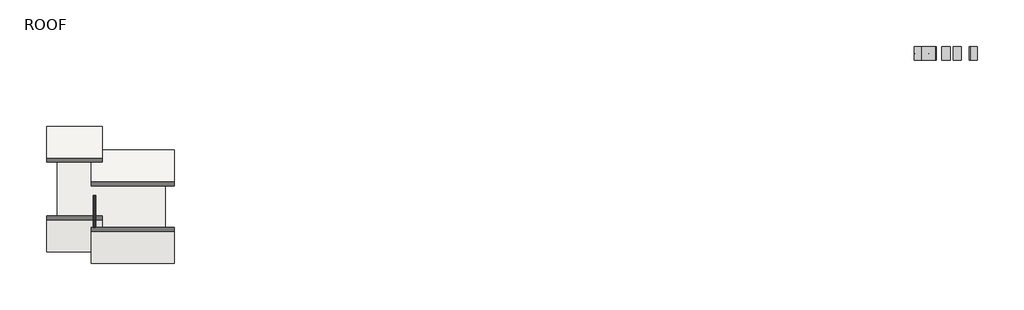
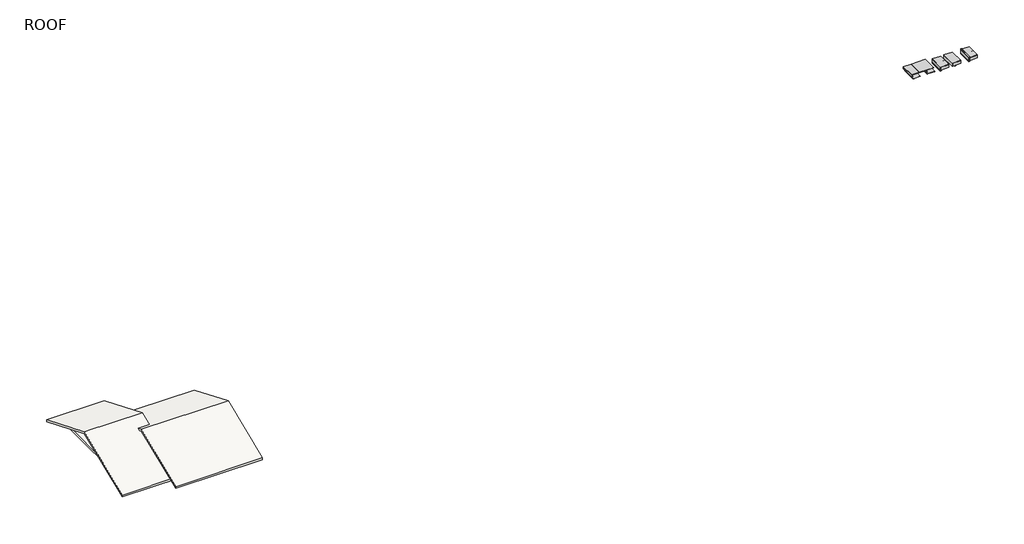
# One storey: 38 proxies, 2 roofs, 1 covering, 1 wall.
"""IFC4 building model written with IfcOpenShell, lengths in millimetres."""

import ifcopenshell
import ifcopenshell.guid

model = None  # the IFC model being written
_history = None  # IfcOwnerHistory: only IFC2X3 demands one
_inside = {}  # id of a spatial element -> (the spatial element, [elements in it])
_under = {}  # id of a project, library or spatial element -> (it, [spatial elements below it])
_declared = {}  # id of a project -> (the project, [libraries it declares])
_typed = {}  # id of a type object -> (the type object, [elements of that type])
_made_of = {}  # id of a material, layer set ... -> (it, [elements and type objects made of it])


def new_model(schema):
    """Start an empty IFC model of exactly this schema.

    Asked for "IFC4X3", IfcOpenShell would pick the latest addendum, in which some entities
    have other attributes; the version numbers below select the first issue.
    IFC2X3 requires an IfcOwnerHistory on every rooted entity: one is made here for all.
    """
    global model, _history
    if schema == "IFC4X3":
        model = ifcopenshell.file(schema_version=(4, 3, 0, 0))
    else:
        model = ifcopenshell.file(schema=schema)
    _inside.clear()
    _under.clear()
    _declared.clear()
    _typed.clear()
    _made_of.clear()
    _history = None
    if model.schema == "IFC2X3":
        org = make("IfcOrganization", Name="unknown")
        user = make(
            "IfcPersonAndOrganization",
            ThePerson=make("IfcPerson", FamilyName="unknown"),
            TheOrganization=org,
        )
        app = make(
            "IfcApplication",
            ApplicationDeveloper=org,
            Version="unknown",
            ApplicationFullName="unknown",
            ApplicationIdentifier="unknown",
        )
        _history = make(
            "IfcOwnerHistory",
            OwningUser=user,
            OwningApplication=app,
            ChangeAction="ADDED",
            CreationDate=0,
        )
    return model


def make(cls, **values):
    """One entity of the class cls with the attributes given. An attribute that is None is left unset."""
    return model.create_entity(
        cls, **{name: value for name, value in values.items() if value is not None}
    )


def rooted(cls, **values):
    """An entity with a GlobalId (a new one), such as an element, a storey or a relation."""
    return make(cls, GlobalId=ifcopenshell.guid.new(), OwnerHistory=_history, **values)


def si_unit(unit_type, name, prefix=None):
    """IfcSIUnit, for example si_unit("LENGTHUNIT", "METRE", prefix="MILLI")."""
    return make("IfcSIUnit", UnitType=unit_type, Prefix=prefix, Name=name)


def assignment(units):
    """IfcUnitAssignment: the units of a project."""
    return None if units is None else make("IfcUnitAssignment", Units=units)


def point(xyz):
    """IfcCartesianPoint."""
    return None if xyz is None else make("IfcCartesianPoint", Coordinates=xyz)


def direction(xyz):
    """IfcDirection."""
    return None if xyz is None else make("IfcDirection", DirectionRatios=xyz)


def frame(location, z_axis=None, x_axis=None):
    """IfcAxis2Placement3D, a coordinate frame: its origin and axes. An axis left out is left unset."""
    return make(
        "IfcAxis2Placement3D",
        Location=point(location),
        Axis=direction(z_axis),
        RefDirection=direction(x_axis),
    )


def origin():
    """The frame at (0, 0, 0) with its axes left unset."""
    return frame((0.0, 0.0, 0.0))


def place(relative_to, where):
    """IfcLocalPlacement: puts the frame where relative to a parent placement (None: the world)."""
    return make(
        "IfcLocalPlacement", PlacementRelTo=relative_to, RelativePlacement=where
    )


def context(
    kind, dimensions, precision=None, world=None, true_north=None, identifier=None
):
    """IfcGeometricRepresentationContext, for example the 3D "Model" context."""
    return make(
        "IfcGeometricRepresentationContext",
        ContextIdentifier=identifier,
        ContextType=kind,
        CoordinateSpaceDimension=dimensions,
        Precision=precision,
        WorldCoordinateSystem=world,
        TrueNorth=true_north,
    )


def project(units=None, contexts=None):
    """IfcProject with its units and contexts."""
    return rooted(
        "IfcProject",
        Name="project",
        RepresentationContexts=contexts,
        UnitsInContext=assignment(units),
    )


def spatial(cls, under=None, at=None, **own):
    """A site, building, storey or space (cls), placed at a placement, below another one or the project."""
    s = rooted(cls, ObjectPlacement=at, **own)
    if under is not None:
        _under.setdefault(under.id(), (under, []))[1].append(s)
    return s


def polyline(points):
    """IfcPolyline through the points."""
    return make("IfcPolyline", Points=[point(p) for p in points])


def outline(outer, holes=None, kind="AREA"):
    """IfcArbitraryClosedProfileDef: a profile drawn as a closed curve; with holes, ...WithVoids."""
    if holes is None:
        return make("IfcArbitraryClosedProfileDef", ProfileType=kind, OuterCurve=outer)
    return make(
        "IfcArbitraryProfileDefWithVoids",
        ProfileType=kind,
        OuterCurve=outer,
        InnerCurves=holes,
    )


def extrude(swept, where, along, depth):
    """IfcExtrudedAreaSolid: the profile swept, set in the frame where, extruded along a direction by depth."""
    return make(
        "IfcExtrudedAreaSolid",
        SweptArea=swept,
        Position=where,
        ExtrudedDirection=direction(along),
        Depth=depth,
    )


def shape(context_of_items, identifier, shape_type, items):
    """IfcShapeRepresentation: the items that make up one representation, for example the "Body"."""
    return make(
        "IfcShapeRepresentation",
        ContextOfItems=context_of_items,
        RepresentationIdentifier=identifier,
        RepresentationType=shape_type,
        Items=items,
    )


def source(mapping_origin, context_of_items, identifier, shape_type, items):
    """IfcRepresentationMap: a shape defined once, which mapped items show again and again."""
    return make(
        "IfcRepresentationMap",
        MappingOrigin=mapping_origin,
        MappedRepresentation=shape(context_of_items, identifier, shape_type, items),
    )


def transform(
    local_origin,
    x_axis=None,
    y_axis=None,
    z_axis=None,
    scale=None,
    scale2=None,
    scale3=None,
    uniform=True,
):
    """IfcCartesianTransformationOperator3D, or its non-uniform kind. x_axis, y_axis, z_axis: its Axis1, 2, 3."""
    if uniform:
        return make(
            "IfcCartesianTransformationOperator3D",
            Axis1=direction(x_axis),
            Axis2=direction(y_axis),
            LocalOrigin=point(local_origin),
            Scale=scale,
            Axis3=direction(z_axis),
        )
    return make(
        "IfcCartesianTransformationOperator3DnonUniform",
        Axis1=direction(x_axis),
        Axis2=direction(y_axis),
        LocalOrigin=point(local_origin),
        Scale=scale,
        Axis3=direction(z_axis),
        Scale2=scale2,
        Scale3=scale3,
    )


def mapped(mapping_source, mapping_target):
    """IfcMappedItem: shows the shape of a source again, moved by a transform."""
    return make(
        "IfcMappedItem", MappingSource=mapping_source, MappingTarget=mapping_target
    )


def made_of(thing, what):
    """Note that an element or type object is made of a material, layer set ...; save() writes the relation."""
    if what is not None:
        _made_of.setdefault(what.id(), (what, []))[1].append(thing)
    return thing


def element(
    cls,
    number,
    at=None,
    inside=None,
    cuts=None,
    type_object=None,
    material=None,
    context=None,
    identifier="Body",
    shape_type=None,
    held_by="IfcProductDefinitionShape",
    body=None,
    shapes=None,
    **own,
):
    """One element of the class cls, such as IfcWall. Its Tag is "e" and its number.

    at: its placement. inside: the storey or other place that contains it. cuts: it is an
    opening in that element (IfcRelVoidsElement). A single representation is given by context,
    identifier, shape_type and body (its items); several are given by shapes. held_by: the class
    of the entity that holds the representations. save() writes the other relations.
    """
    e = rooted(cls, Tag="e%d" % number, ObjectPlacement=at, **own)
    if body is not None:
        shapes = [shape(context, identifier, shape_type, body)]
    if shapes is not None:
        e.Representation = make(held_by, Representations=shapes)
    if inside is not None:
        _inside.setdefault(inside.id(), (inside, []))[1].append(e)
    if cuts is not None:
        rooted(
            "IfcRelVoidsElement", RelatingBuildingElement=cuts, RelatedOpeningElement=e
        )
    if type_object is not None:
        _typed.setdefault(type_object.id(), (type_object, []))[1].append(e)
    return made_of(e, material)


def aggregate(whole, parts):
    """IfcRelAggregates: a whole, such as a stair, and the parts it consists of."""
    return rooted("IfcRelAggregates", RelatingObject=whole, RelatedObjects=parts)


def save(model, path):
    """Write the relations noted so far, then the file.

    IfcRelAggregates (storeys below a building ...), IfcRelContainedInSpatialStructure (elements
    in a storey), IfcRelDefinesByType, IfcRelAssociatesMaterial and IfcRelDeclares: one each for
    every whole, place, type object, material and project.
    """
    for whole, parts in _under.values():
        aggregate(whole, parts)
    for where, things in _inside.values():
        rooted(
            "IfcRelContainedInSpatialStructure",
            RelatedElements=things,
            RelatingStructure=where,
        )
    for kind, things in _typed.values():
        rooted("IfcRelDefinesByType", RelatedObjects=things, RelatingType=kind)
    for what, things in _made_of.values():
        rooted("IfcRelAssociatesMaterial", RelatedObjects=things, RelatingMaterial=what)
    for by, libraries in _declared.values():
        rooted("IfcRelDeclares", RelatingContext=by, RelatedDefinitions=libraries)
    model.write(path)


def generic_models_10_generic_models_1_ea081297(model_context):
    return source(origin(), model_context, "Body", "SweptSolid", [
        extrude(outline(polyline([(49758.6, 0.0), (49720.5, 0.0), (49720.5, 1219.2), (49758.6, 1219.2), (49758.6, 0.0)])), frame((0.0, 0.0, 5507.83125), z_axis=(0.0, 0.0, 1.0), x_axis=(1.0, 0.0, 0.0)), (0.0, 0.0, 1.0), 139.7),
    ])


def generic_models_109_generic_models_1_8619d77b(model_context):
    return source(origin(), model_context, "Body", "SweptSolid", [
        extrude(outline(polyline([(51003.2, 0.0), (50914.3, 0.0), (50914.3, 1219.2), (51003.2, 1219.2), (51003.2, 0.0)])), frame((0.0, 0.0, 5184.378125), z_axis=(0.0, 0.0, 1.0), x_axis=(1.0, 0.0, 0.0)), (0.0, 0.0, 1.0), 38.1),
    ])


def generic_models_110_generic_models_1_6bdce9b6(model_context):
    return source(origin(), model_context, "Body", "SweptSolid", [
        extrude(outline(polyline([(51642.1451407, 1219.2), (51642.1451407, 0.0), (50914.3, 0.0), (50914.3, 1219.2), (51642.1451407, 1219.2)])), frame((0.0, 0.0, 5508.228125), z_axis=(0.0, 0.0, 1.0), x_axis=(1.0, 0.0, 0.0)), (0.0, 0.0, 1.0), 19.05),
    ])


def generic_models_112_generic_models_65_d168d7b0(model_context):
    return source(origin(), model_context, "Body", "SweptSolid", [
        extrude(outline(polyline([(50952.4, 592.1375), (50952.4, 630.2375), (51642.1451407, 630.2375), (51642.1451407, 592.1375), (50952.4, 592.1375)])), frame((0.0, 0.0, 5222.478125), z_axis=(0.0, 0.0, 1.0), x_axis=(1.0, 0.0, 0.0)), (0.0, 0.0, 1.0), 285.75),
    ])


def generic_models_113_generic_models_1_101608ab(model_context):
    return source(origin(), model_context, "Body", "SweptSolid", [
        extrude(outline(polyline([(52171.6, 0.0), (52133.5, 0.0), (52133.5, 1219.2), (52171.6, 1219.2), (52171.6, 0.0)])), frame((0.0, 0.0, 5222.478125), z_axis=(0.0, 0.0, 1.0), x_axis=(1.0, 0.0, 0.0)), (0.0, 0.0, 1.0), 285.75),
    ])


def generic_models_114_generic_models_1_a6fb1c2c(model_context):
    return source(origin(), model_context, "Body", "SweptSolid", [
        extrude(outline(polyline([(51642.1451407, 1219.2), (51642.1451407, 0.0), (50965.9242022, 0.0), (50965.9242022, 1219.2), (51642.1451407, 1219.2)])), frame((0.0, 0.0, 5237.6235034), z_axis=(0.0, 0.0, 1.0), x_axis=(1.0, 0.0, 0.0)), (0.0, 0.0, 1.0), 254.0),
    ])


def generic_models_12_generic_models_46_b8a9a4e8(model_context):
    return source(origin(), model_context, "Body", "SweptSolid", [
        extrude(outline(polyline([(49757.8505137, 0.0), (49721.1284797, 0.0), (49721.1284797, 1219.2), (49757.8505137, 1219.2), (49757.8505137, 0.0)])), frame((0.0, 0.0, 5505.7509163), z_axis=(0.0, 0.0, 1.0), x_axis=(1.0, 0.0, 0.0)), (0.0, 0.0, 1.0), 1.5875),
    ])


def generic_models_13_generic_models_65_9e643fb9(model_context):
    return source(origin(), model_context, "Body", "SweptSolid", [
        extrude(outline(polyline([(49128.3625, 592.1375), (49128.3625, 630.2375), (50347.5625, 630.2375), (50347.5625, 592.1375), (49128.3625, 592.1375)])), frame((0.0, 0.0, 5507.83125), z_axis=(0.0, 0.0, 1.0), x_axis=(1.0, 0.0, 0.0)), (0.0, 0.0, 1.0), 139.7),
    ])


def generic_models_14_generic_models_1_e8c90d4c(model_context):
    return source(origin(), model_context, "Body", "SweptSolid", [
        extrude(outline(polyline([(2277.1204978, 49799.875), (2239.0204978, 49799.875), (2239.0204978, 49825.275), (2240.6079978, 49825.275), (2240.6079978, 49801.4625), (2277.1204978, 49801.4625), (2277.1204978, 49799.875)])), frame((0.0, 0.0, 0.0), z_axis=(0.0, 1.0, 0.0), x_axis=(0.0, 0.0, 1.0)), (0.0, 0.0, 1.0), 1219.2),
    ])


def generic_models_22_generic_models_1_e5767157(model_context):
    return source(origin(), model_context, "Body", "SweptSolid", [
        extrude(outline(polyline([(2409.6091, 49800.66875), (2409.6091, 49799.875), (2407.0592364, 49799.875), (2405.4618473, 49749.075), (2404.6631527, 49749.075), (2403.0657636, 49799.875), (2400.5159, 49799.875), (2400.5159, 49800.66875), (2409.6091, 49800.66875)])), frame((0.0, 565.15, 0.0), z_axis=(0.0, 1.0, 0.0), x_axis=(0.0, 0.0, 1.0)), (0.0, 0.0, 1.0), 12.7),
    ])


def generic_models_226_generic_models_1_7dc37832(model_context):
    return source(origin(), model_context, "Body", "SweptSolid", [
        extrude(outline(polyline([(5263.35625, 49733.4159), (5263.35625, 49742.5091), (5264.15, 49742.5091), (5264.15, 49739.9592364), (5314.95, 49738.3618473), (5314.95, 49737.5631527), (5264.15, 49735.9657636), (5264.15, 49733.4159), (5263.35625, 49733.4159)])), frame((0.0, 565.15, 0.0), z_axis=(0.0, 1.0, 0.0), x_axis=(0.0, 0.0, 1.0)), (0.0, 0.0, 1.0), 12.7),
    ])


def generic_models_202_generic_models_1_0ad20a8b(model_context):
    return source(origin(), model_context, "Body", "SweptSolid", [
        extrude(outline(polyline([(2253.330428, 49813.3451407), (2242.217928, 49813.3451407), (2242.217928, 49826.0451407), (2234.280428, 49828.9341545), (2234.280428, 50422.9451407), (2253.330428, 50422.9451407), (2253.330428, 49813.3451407)])), frame((0.0, 0.0, 0.0), z_axis=(0.0, 1.0, 0.0), x_axis=(0.0, 0.0, 1.0)), (0.0, 0.0, 1.0), 1219.2),
    ])


def generic_models_233_generic_models_1_ae5bae41(model_context):
    return source(origin(), model_context, "Body", "SweptSolid", [
        extrude(outline(polyline([(48564.8, 0.0), (48475.9, 0.0), (48475.9, 1219.2), (48564.8, 1219.2), (48564.8, 0.0)])), frame((0.0, 0.0, 5467.35), z_axis=(0.0, 0.0, 1.0), x_axis=(1.0, 0.0, 0.0)), (0.0, 0.0, 1.0), 38.1),
    ])


def generic_models_236_generic_models_1_f8917e71(model_context):
    return source(origin(), model_context, "Body", "SweptSolid", [
        extrude(outline(polyline([(48507.65, 0.0), (48469.55, 0.0), (48469.55, 1219.2), (48507.65, 1219.2), (48507.65, 0.0)])), frame((0.0, 0.0, 5507.83125), z_axis=(0.0, 0.0, 1.0), x_axis=(1.0, 0.0, 0.0)), (0.0, 0.0, 1.0), 139.7),
    ])


def generic_models_237_generic_models_65_1df05f16(model_context):
    return source(origin(), model_context, "Body", "SweptSolid", [
        extrude(outline(polyline([(48469.55, 592.1375), (48469.55, 630.2375), (49128.3625, 630.2375), (49128.3625, 592.1375), (48469.55, 592.1375)])), frame((0.0, 0.0, 5507.83125), z_axis=(0.0, 0.0, 1.0), x_axis=(1.0, 0.0, 0.0)), (0.0, 0.0, 1.0), 139.7),
    ])


def generic_models_239_generic_models_46_95e6735a(model_context):
    return source(origin(), model_context, "Body", "SweptSolid", [
        extrude(outline(polyline([(50347.5625, 0.0), (49691.4320511, 0.0), (49691.4320511, 1219.2), (50347.5625, 1219.2), (50347.5625, 0.0)])), frame((0.0, 0.0, 5505.7509163), z_axis=(0.0, 0.0, 1.0), x_axis=(1.0, 0.0, 0.0)), (0.0, 0.0, 1.0), 1.5875),
    ])


def generic_models_240_generic_models_1_611786cf(model_context):
    return source(origin(), model_context, "Body", "SweptSolid", [
        extrude(outline(polyline([(49128.3625, 1219.2), (49128.3625, 0.0), (48469.55, 0.0), (48469.55, 1219.2), (49128.3625, 1219.2)])), frame((0.0, 0.0, 5649.9125), z_axis=(0.0, 0.0, 1.0), x_axis=(1.0, 0.0, 0.0)), (0.0, 0.0, 1.0), 19.05),
    ])


def generic_models_29_generic_models_1_59087225(model_context):
    return source(origin(), model_context, "Body", "SweptSolid", [
        extrude(outline(polyline([(50347.5625, 1219.2), (50347.5625, 0.0), (49128.3625, 0.0), (49128.3625, 1219.2), (50347.5625, 1219.2)])), frame((0.0, 0.0, 5647.53125), z_axis=(0.0, 0.0, 1.0), x_axis=(1.0, 0.0, 0.0)), (0.0, 0.0, 1.0), 19.05),
    ])


def generic_models_37_generic_models_1_916dd7c6(model_context):
    return source(origin(), model_context, "Body", "SweptSolid", [
        extrude(outline(polyline([(2409.6091, 49675.25625), (2400.5159, 49675.25625), (2400.5159, 49676.05), (2403.0657636, 49676.05), (2404.6631527, 49726.85), (2405.4618473, 49726.85), (2407.0592364, 49676.05), (2409.6091, 49676.05), (2409.6091, 49675.25625)])), frame((0.0, 565.15, 0.0), z_axis=(0.0, 1.0, 0.0), x_axis=(0.0, 0.0, 1.0)), (0.0, 0.0, 1.0), 12.7),
    ])


def generic_models_103_generic_models_1_250a6a11(model_context):
    return source(origin(), model_context, "Body", "SweptSolid", [
        extrude(outline(polyline([(49784.0, 0.0), (49695.1, 0.0), (49695.1, 1219.2), (49784.0, 1219.2), (49784.0, 0.0)])), frame((0.0, 0.0, 5264.15), z_axis=(0.0, 0.0, 1.0), x_axis=(1.0, 0.0, 0.0)), (0.0, 0.0, 1.0), 38.1),
    ])


def generic_models_71_generic_models_1_508a995f(model_context):
    return source(origin(), model_context, "Body", "SweptSolid", [
        extrude(outline(polyline([(50952.4, 0.0), (50914.3, 0.0), (50914.3, 1219.2), (50952.4, 1219.2), (50952.4, 0.0)])), frame((0.0, 0.0, 5222.478125), z_axis=(0.0, 0.0, 1.0), x_axis=(1.0, 0.0, 0.0)), (0.0, 0.0, 1.0), 285.75),
    ])


def generic_models_87_generic_models_1_55a64953(model_context):
    return source(origin(), model_context, "Body", "SweptSolid", [
        extrude(outline(polyline([(51968.4, 0.0), (51930.3, 0.0), (51930.3, 1219.2), (51968.4, 1219.2), (51968.4, 0.0)])), frame((0.0, 0.0, 5222.478125), z_axis=(0.0, 0.0, 1.0), x_axis=(1.0, 0.0, 0.0)), (0.0, 0.0, 1.0), 285.75),
    ])


model = new_model("IFC4")

# Units and contexts
model_context = context("Model", 3, world=origin())
ifc_project = project(units=[si_unit("LENGTHUNIT", "METRE", prefix="MILLI")], contexts=[model_context])

# Site, building, storey
site = spatial("IfcSite", under=ifc_project)
building = spatial("IfcBuilding", under=site)
storey = spatial("IfcBuildingStorey", under=building, Name="ROOF", Elevation=5130.8)

# Proxies
placement = place(None, origin())
generic_models_10_generic_models_1_shape = generic_models_10_generic_models_1_ea081297(model_context)
element("IfcBuildingElementProxy", 1, Name="Generic Models 10 : Generic Models 1", ObjectType="Generic Models 10 : Generic Models 1", at=placement, inside=storey, context=model_context, shape_type="MappedRepresentation", body=[
    mapped(generic_models_10_generic_models_1_shape, transform((0.0, 0.0, 0.0), x_axis=(1.0, 0.0, 0.0), y_axis=(0.0, 1.0, 0.0), z_axis=(0.0, 0.0, 1.0))),
])
generic_models_109_generic_models_1_shape = generic_models_109_generic_models_1_8619d77b(model_context)
element("IfcBuildingElementProxy", 2, Name="Generic Models 109 : Generic Models 1", ObjectType="Generic Models 109 : Generic Models 1", at=placement, inside=storey, context=model_context, shape_type="MappedRepresentation", body=[
    mapped(generic_models_109_generic_models_1_shape, transform((2438.4, 0.0, 0.0), x_axis=(1.0, 0.0, 0.0), y_axis=(0.0, 1.0, 0.0), z_axis=(0.0, 0.0, 1.0))),
])
generic_models_110_generic_models_1_shape = generic_models_110_generic_models_1_6bdce9b6(model_context)
element("IfcBuildingElementProxy", 3, Name="Generic Models 110 : Generic Models 1", ObjectType="Generic Models 110 : Generic Models 1", at=placement, inside=storey, context=model_context, shape_type="MappedRepresentation", body=[
    mapped(generic_models_110_generic_models_1_shape, transform((2438.4, 0.0, 0.0), x_axis=(1.0, 0.0, 0.0), y_axis=(0.0, 1.0, 0.0), z_axis=(0.0, 0.0, 1.0))),
])
element("IfcBuildingElementProxy", 4, Name="Generic Models 111 : Generic Models 1", ObjectType="Generic Models 111 : Generic Models 1", at=placement, inside=storey, context=model_context, shape_type="MappedRepresentation", body=[
    mapped(generic_models_109_generic_models_1_shape, transform((2438.4, 0.0, -38.1), x_axis=(1.0, 0.0, 0.0), y_axis=(0.0, 1.0, 0.0), z_axis=(0.0, 0.0, 1.0))),
])
generic_models_112_generic_models_65_shape = generic_models_112_generic_models_65_d168d7b0(model_context)
element("IfcBuildingElementProxy", 5, Name="Generic Models 112 : Generic Models 65", ObjectType="Generic Models 112 : Generic Models 65", at=placement, inside=storey, context=model_context, shape_type="MappedRepresentation", body=[
    mapped(generic_models_112_generic_models_65_shape, transform((2438.4, 0.0, 0.0), x_axis=(1.0, 0.0, 0.0), y_axis=(0.0, 1.0, 0.0), z_axis=(0.0, 0.0, 1.0))),
])
generic_models_113_generic_models_1_shape = generic_models_113_generic_models_1_101608ab(model_context)
element("IfcBuildingElementProxy", 6, Name="Generic Models 113 : Generic Models 1", ObjectType="Generic Models 113 : Generic Models 1", at=placement, inside=storey, context=model_context, shape_type="MappedRepresentation", body=[
    mapped(generic_models_113_generic_models_1_shape, transform((1219.2, 0.0, 0.0), x_axis=(1.0, 0.0, 0.0), y_axis=(0.0, 1.0, 0.0), z_axis=(0.0, 0.0, 1.0))),
])
generic_models_114_generic_models_1_shape = generic_models_114_generic_models_1_a6fb1c2c(model_context)
element("IfcBuildingElementProxy", 7, Name="Generic Models 114 : Generic Models 1", ObjectType="Generic Models 114 : Generic Models 1", at=placement, inside=storey, context=model_context, shape_type="MappedRepresentation", body=[
    mapped(generic_models_114_generic_models_1_shape, transform((2438.4, 0.0, 0.0), x_axis=(1.0, 0.0, 0.0), y_axis=(0.0, 1.0, 0.0), z_axis=(0.0, 0.0, 1.0))),
])
element("IfcBuildingElementProxy", 8, Name="Generic Models 115 : Generic Models 1", ObjectType="Generic Models 115 : Generic Models 1", at=placement, inside=storey, context=model_context, shape_type="MappedRepresentation", body=[
    mapped(generic_models_109_generic_models_1_shape, transform((2438.4, 0.0, 342.9), x_axis=(1.0, 0.0, 0.0), y_axis=(0.0, 1.0, 0.0), z_axis=(0.0, 0.0, 1.0))),
])
generic_models_12_generic_models_46_shape = generic_models_12_generic_models_46_b8a9a4e8(model_context)
element("IfcBuildingElementProxy", 9, Name="Generic Models 12 : Generic Models 46", ObjectType="Generic Models 12 : Generic Models 46", at=placement, inside=storey, context=model_context, shape_type="MappedRepresentation", body=[
    mapped(generic_models_12_generic_models_46_shape, transform((0.0, 0.0, 0.0), x_axis=(1.0, 0.0, 0.0), y_axis=(0.0, 1.0, 0.0), z_axis=(0.0, 0.0, 1.0))),
])
generic_models_13_generic_models_65_shape = generic_models_13_generic_models_65_9e643fb9(model_context)
element("IfcBuildingElementProxy", 10, Name="Generic Models 13 : Generic Models 65", ObjectType="Generic Models 13 : Generic Models 65", at=placement, inside=storey, context=model_context, shape_type="MappedRepresentation", body=[
    mapped(generic_models_13_generic_models_65_shape, transform((0.0, 0.0, 0.0), x_axis=(1.0, 0.0, 0.0), y_axis=(0.0, 1.0, 0.0), z_axis=(0.0, 0.0, 1.0))),
])
generic_models_14_generic_models_1_shape = generic_models_14_generic_models_1_e8c90d4c(model_context)
element("IfcBuildingElementProxy", 11, Name="Generic Models 14 : Generic Models 1", ObjectType="Generic Models 14 : Generic Models 1", at=placement, inside=storey, context=model_context, shape_type="MappedRepresentation", body=[
    mapped(generic_models_14_generic_models_1_shape, transform((0.0, 0.0, 3050.778125), x_axis=(1.0, 0.0, 0.0), y_axis=(0.0, 1.0, 0.0), z_axis=(0.0, 0.0, 1.0))),
])
generic_models_22_generic_models_1_shape = generic_models_22_generic_models_1_e5767157(model_context)
element("IfcBuildingElementProxy", 12, Name="Generic Models 22 : Generic Models 1", ObjectType="Generic Models 22 : Generic Models 1", at=placement, inside=storey, context=model_context, shape_type="MappedRepresentation", body=[
    mapped(generic_models_22_generic_models_1_shape, transform((0.0, 0.0, 3081.3375), x_axis=(1.0, 0.0, 0.0), y_axis=(0.0, 1.0, 0.0), z_axis=(0.0, 0.0, 1.0))),
])
element("IfcBuildingElementProxy", 13, Name="Generic Models 224 : Generic Models 1", ObjectType="Generic Models 224 : Generic Models 1", at=placement, inside=storey, context=model_context, shape_type="MappedRepresentation", body=[
    mapped(generic_models_14_generic_models_1_shape, transform((-1217.6125, 0.0, 3050.778125), x_axis=(1.0, 0.0, 0.0), y_axis=(0.0, 1.0, 0.0), z_axis=(0.0, 0.0, 1.0))),
])
element("IfcBuildingElementProxy", 14, Name="Generic Models 225 : Generic Models 1", ObjectType="Generic Models 225 : Generic Models 1", at=placement, inside=storey, context=model_context, shape_type="MappedRepresentation", body=[
    mapped(generic_models_22_generic_models_1_shape, transform((-1219.2, 0.0, 3081.3375), x_axis=(1.0, 0.0, 0.0), y_axis=(0.0, 1.0, 0.0), z_axis=(0.0, 0.0, 1.0))),
])
generic_models_226_generic_models_1_shape = generic_models_226_generic_models_1_7dc37832(model_context)
element("IfcBuildingElementProxy", 15, Name="Generic Models 226 : Generic Models 1", ObjectType="Generic Models 226 : Generic Models 1", at=placement, inside=storey, context=model_context, shape_type="MappedRepresentation", body=[
    mapped(generic_models_226_generic_models_1_shape, transform((-1219.2, 0.0, 203.2), x_axis=(1.0, 0.0, 0.0), y_axis=(0.0, 1.0, 0.0), z_axis=(0.0, 0.0, 1.0))),
])
generic_models_202_generic_models_1_shape = generic_models_202_generic_models_1_0ad20a8b(model_context)
element("IfcBuildingElementProxy", 16, Name="Generic Models 231 : Generic Models 1", ObjectType="Generic Models 231 : Generic Models 1", at=placement, inside=storey, context=model_context, shape_type="MappedRepresentation", body=[
    mapped(generic_models_202_generic_models_1_shape, transform((-1217.6125, 0.0, 3050.778125), x_axis=(1.0, 0.0, 0.0), y_axis=(0.0, 1.0, 0.0), z_axis=(0.0, 0.0, 1.0))),
])
generic_models_233_generic_models_1_shape = generic_models_233_generic_models_1_ae5bae41(model_context)
element("IfcBuildingElementProxy", 17, Name="Generic Models 233 : Generic Models 1", ObjectType="Generic Models 233 : Generic Models 1", at=placement, inside=storey, context=model_context, shape_type="MappedRepresentation", body=[
    mapped(generic_models_233_generic_models_1_shape, transform((0.0, 0.0, 0.0), x_axis=(1.0, 0.0, 0.0), y_axis=(0.0, 1.0, 0.0), z_axis=(0.0, 0.0, 1.0))),
])
generic_models_236_generic_models_1_shape = generic_models_236_generic_models_1_f8917e71(model_context)
element("IfcBuildingElementProxy", 18, Name="Generic Models 236 : Generic Models 1", ObjectType="Generic Models 236 : Generic Models 1", at=placement, inside=storey, context=model_context, shape_type="MappedRepresentation", body=[
    mapped(generic_models_236_generic_models_1_shape, transform((0.0, 0.0, 0.0), x_axis=(1.0, 0.0, 0.0), y_axis=(0.0, 1.0, 0.0), z_axis=(0.0, 0.0, 1.0))),
])
generic_models_237_generic_models_65_shape = generic_models_237_generic_models_65_1df05f16(model_context)
element("IfcBuildingElementProxy", 19, Name="Generic Models 237 : Generic Models 65", ObjectType="Generic Models 237 : Generic Models 65", at=placement, inside=storey, context=model_context, shape_type="MappedRepresentation", body=[
    mapped(generic_models_237_generic_models_65_shape, transform((0.0, 0.0, 0.0), x_axis=(1.0, 0.0, 0.0), y_axis=(0.0, 1.0, 0.0), z_axis=(0.0, 0.0, 1.0))),
])
generic_models_239_generic_models_46_shape = generic_models_239_generic_models_46_95e6735a(model_context)
element("IfcBuildingElementProxy", 20, Name="Generic Models 239 : Generic Models 46", ObjectType="Generic Models 239 : Generic Models 46", at=placement, inside=storey, context=model_context, shape_type="MappedRepresentation", body=[
    mapped(generic_models_239_generic_models_46_shape, transform((-1219.2, 0.0, 142.08125), x_axis=(1.0, 0.0, 0.0), y_axis=(0.0, 1.0, 0.0), z_axis=(0.0, 0.0, 1.0))),
])
generic_models_240_generic_models_1_shape = generic_models_240_generic_models_1_611786cf(model_context)
element("IfcBuildingElementProxy", 21, Name="Generic Models 240 : Generic Models 1", ObjectType="Generic Models 240 : Generic Models 1", at=placement, inside=storey, context=model_context, shape_type="MappedRepresentation", body=[
    mapped(generic_models_240_generic_models_1_shape, transform((0.0, 0.0, 0.0), x_axis=(1.0, 0.0, 0.0), y_axis=(0.0, 1.0, 0.0), z_axis=(0.0, 0.0, 1.0))),
])
element("IfcBuildingElementProxy", 22, Name="Generic Models 25 : Generic Models 46", ObjectType="Generic Models 25 : Generic Models 46", at=placement, inside=storey, context=model_context, shape_type="MappedRepresentation", body=[
    mapped(generic_models_12_generic_models_46_shape, transform((0.0, 0.0, 142.08125), x_axis=(1.0, 0.0, 0.0), y_axis=(0.0, 1.0, 0.0), z_axis=(0.0, 0.0, 1.0))),
])
generic_models_29_generic_models_1_shape = generic_models_29_generic_models_1_59087225(model_context)
element("IfcBuildingElementProxy", 23, Name="Generic Models 29 : Generic Models 1", ObjectType="Generic Models 29 : Generic Models 1", at=placement, inside=storey, context=model_context, shape_type="MappedRepresentation", body=[
    mapped(generic_models_29_generic_models_1_shape, transform((0.0, 0.0, 2.38125), x_axis=(1.0, 0.0, 0.0), y_axis=(0.0, 1.0, 0.0), z_axis=(0.0, 0.0, 1.0))),
])
element("IfcBuildingElementProxy", 24, Name="Generic Models 39 : Generic Models 1", ObjectType="Generic Models 39 : Generic Models 1", at=placement, inside=storey, context=model_context, shape_type="MappedRepresentation", body=[
    mapped(generic_models_226_generic_models_1_shape, transform((0.0, 0.0, 203.2), x_axis=(1.0, 0.0, 0.0), y_axis=(0.0, 1.0, 0.0), z_axis=(0.0, 0.0, 1.0))),
])
generic_models_37_generic_models_1_shape = generic_models_37_generic_models_1_916dd7c6(model_context)
element("IfcBuildingElementProxy", 25, Name="Generic Models 47 : Generic Models 1", ObjectType="Generic Models 47 : Generic Models 1", at=placement, inside=storey, context=model_context, shape_type="MappedRepresentation", body=[
    mapped(generic_models_37_generic_models_1_shape, transform((3.175, 0.0, 3081.3375), x_axis=(1.0, 0.0, 0.0), y_axis=(0.0, 1.0, 0.0), z_axis=(0.0, 0.0, 1.0))),
])
element("IfcBuildingElementProxy", 26, Name="Generic Models 49 : Generic Models 1", ObjectType="Generic Models 49 : Generic Models 1", at=placement, inside=storey, context=model_context, shape_type="MappedRepresentation", body=[
    mapped(generic_models_202_generic_models_1_shape, transform((0.0, 0.0, 3050.778125), x_axis=(1.0, 0.0, 0.0), y_axis=(0.0, 1.0, 0.0), z_axis=(0.0, 0.0, 1.0))),
])
element("IfcBuildingElementProxy", 27, Name="Generic Models 59 : Generic Models 65", ObjectType="Generic Models 59 : Generic Models 65", at=placement, inside=storey, context=model_context, shape_type="MappedRepresentation", body=[
    mapped(generic_models_112_generic_models_65_shape, transform((0.0, 0.0, 0.0), x_axis=(1.0, 0.0, 0.0), y_axis=(0.0, 1.0, 0.0), z_axis=(0.0, 0.0, 1.0))),
])
generic_models_103_generic_models_1_shape = generic_models_103_generic_models_1_250a6a11(model_context)
element("IfcBuildingElementProxy", 28, Name="Generic Models 6 : Generic Models 1", ObjectType="Generic Models 6 : Generic Models 1", at=placement, inside=storey, context=model_context, shape_type="MappedRepresentation", body=[
    mapped(generic_models_103_generic_models_1_shape, transform((0.0, 0.0, 203.2), x_axis=(1.0, 0.0, 0.0), y_axis=(0.0, 1.0, 0.0), z_axis=(0.0, 0.0, 1.0))),
])
element("IfcBuildingElementProxy", 29, Name="Generic Models 64 : Generic Models 1", ObjectType="Generic Models 64 : Generic Models 1", at=placement, inside=storey, context=model_context, shape_type="MappedRepresentation", body=[
    mapped(generic_models_109_generic_models_1_shape, transform((0.0, 0.0, 0.0), x_axis=(1.0, 0.0, 0.0), y_axis=(0.0, 1.0, 0.0), z_axis=(0.0, 0.0, 1.0))),
])
element("IfcBuildingElementProxy", 30, Name="Generic Models 66 : Generic Models 1", ObjectType="Generic Models 66 : Generic Models 1", at=placement, inside=storey, context=model_context, shape_type="MappedRepresentation", body=[
    mapped(generic_models_110_generic_models_1_shape, transform((0.0, 0.0, 0.0), x_axis=(1.0, 0.0, 0.0), y_axis=(0.0, 1.0, 0.0), z_axis=(0.0, 0.0, 1.0))),
])
element("IfcBuildingElementProxy", 31, Name="Generic Models 70 : Generic Models 1", ObjectType="Generic Models 70 : Generic Models 1", at=placement, inside=storey, context=model_context, shape_type="MappedRepresentation", body=[
    mapped(generic_models_109_generic_models_1_shape, transform((0.0, 0.0, -38.1), x_axis=(1.0, 0.0, 0.0), y_axis=(0.0, 1.0, 0.0), z_axis=(0.0, 0.0, 1.0))),
])
generic_models_71_generic_models_1_shape = generic_models_71_generic_models_1_508a995f(model_context)
element("IfcBuildingElementProxy", 32, Name="Generic Models 71 : Generic Models 1", ObjectType="Generic Models 71 : Generic Models 1", at=placement, inside=storey, context=model_context, shape_type="MappedRepresentation", body=[
    mapped(generic_models_71_generic_models_1_shape, transform((0.0, 0.0, 0.0), x_axis=(1.0, 0.0, 0.0), y_axis=(0.0, 1.0, 0.0), z_axis=(0.0, 0.0, 1.0))),
])
element("IfcBuildingElementProxy", 33, Name="Generic Models 72 : Generic Models 1", ObjectType="Generic Models 72 : Generic Models 1", at=placement, inside=storey, context=model_context, shape_type="MappedRepresentation", body=[
    mapped(generic_models_114_generic_models_1_shape, transform((0.0, 0.0, 0.0), x_axis=(1.0, 0.0, 0.0), y_axis=(0.0, 1.0, 0.0), z_axis=(0.0, 0.0, 1.0))),
])
element("IfcBuildingElementProxy", 34, Name="Generic Models 81 : Generic Models 1", ObjectType="Generic Models 81 : Generic Models 1", at=placement, inside=storey, context=model_context, shape_type="MappedRepresentation", body=[
    mapped(generic_models_109_generic_models_1_shape, transform((1219.2, 0.0, 0.0), x_axis=(1.0, 0.0, 0.0), y_axis=(0.0, 1.0, 0.0), z_axis=(0.0, 0.0, 1.0))),
])
element("IfcBuildingElementProxy", 35, Name="Generic Models 82 : Generic Models 1", ObjectType="Generic Models 82 : Generic Models 1", at=placement, inside=storey, context=model_context, shape_type="MappedRepresentation", body=[
    mapped(generic_models_110_generic_models_1_shape, transform((1016.0, 0.0, 0.0), x_axis=(1.0, 0.0, 0.0), y_axis=(0.0, 1.0, 0.0), z_axis=(0.0, 0.0, 1.0))),
])
element("IfcBuildingElementProxy", 36, Name="Generic Models 86 : Generic Models 65", ObjectType="Generic Models 86 : Generic Models 65", at=placement, inside=storey, context=model_context, shape_type="MappedRepresentation", body=[
    mapped(generic_models_112_generic_models_65_shape, transform((1016.0, 0.0, 0.0), x_axis=(1.0, 0.0, 0.0), y_axis=(0.0, 1.0, 0.0), z_axis=(0.0, 0.0, 1.0))),
])
generic_models_87_generic_models_1_shape = generic_models_87_generic_models_1_55a64953(model_context)
element("IfcBuildingElementProxy", 37, Name="Generic Models 87 : Generic Models 1", ObjectType="Generic Models 87 : Generic Models 1", at=placement, inside=storey, context=model_context, shape_type="MappedRepresentation", body=[
    mapped(generic_models_87_generic_models_1_shape, transform((0.0, 0.0, 0.0), x_axis=(1.0, 0.0, 0.0), y_axis=(0.0, 1.0, 0.0), z_axis=(0.0, 0.0, 1.0))),
])
element("IfcBuildingElementProxy", 38, Name="Generic Models 88 : Generic Models 1", ObjectType="Generic Models 88 : Generic Models 1", at=placement, inside=storey, context=model_context, shape_type="MappedRepresentation", body=[
    mapped(generic_models_114_generic_models_1_shape, transform((1016.0, 0.0, 0.0), x_axis=(1.0, 0.0, 0.0), y_axis=(0.0, 1.0, 0.0), z_axis=(0.0, 0.0, 1.0))),
])

# Covering
element("IfcCovering", 39, ObjectType="GYP. BD WITH INSULATION", at=placement, inside=storey, context=model_context, shape_type="SweptSolid", body=[
    extrude(outline(polyline([(-27692.0039763, -15574.6780399), (-27692.0039763, -7009.6570712), (-24655.1164763, -7009.6570712), (-24655.1164763, -8838.4570712), (-18090.8039763, -8838.4570712), (-18090.8039763, -17403.4780399), (-23577.2039763, -17403.4780399), (-23577.2039763, -15574.6780399), (-27692.0039763, -15574.6780399)])), frame((0.0, 0.0, 5130.8), z_axis=(0.0, 0.0, 1.0), x_axis=(1.0, 0.0, 0.0)), (0.0, 0.0, 1.0), 180.975),
])

# Roofs
element("IfcRoof", 40, ObjectType="Generic - 6\"", at=placement, inside=storey, context=model_context, shape_type="SweptSolid", body=[
    extrude(outline(polyline([(-17064.8820712, 5168.9), (-11480.0570712, 7495.9104167), (-5895.2320712, 5168.9), (-5895.2320712, 5003.8), (-11480.0570712, 7330.8104167), (-17064.8820712, 5003.8), (-17064.8820712, 5168.9)])), frame((-28627.0414763, 0.0, 0.0), z_axis=(1.0, 0.0, 0.0), x_axis=(0.0, 1.0, 0.0)), (0.0, 0.0, 1.0), 4933.95),
])
element("IfcRoof", 41, ObjectType="Generic - 6\"", at=placement, inside=storey, context=model_context, shape_type="SweptSolid", body=[
    extrude(outline(polyline([(-18074.5320712, 5168.9), (-13038.9820712, 7267.0458333), (-8003.4320712, 5168.9), (-8003.4320712, 5003.8), (-13038.9820712, 7101.9458333), (-18074.5320712, 5003.8), (-18074.5320712, 5168.9)])), frame((-24664.6414763, 0.0, 0.0), z_axis=(1.0, 0.0, 0.0), x_axis=(0.0, 1.0, 0.0)), (0.0, 0.0, 1.0), 7385.05),
])

# Wall
element("IfcWall", 42, ObjectType="Upper Wall", at=placement, inside=storey, context=model_context, shape_type="SweptSolid", body=[
    extrude(outline(polyline([(-12035.6820712, 5130.8), (-16655.3070712, 5130.8), (-16655.3070712, 5174.45625), (-16744.2070712, 5174.45625), (-16744.2070712, 5558.1020833), (-13038.9820712, 7101.9458333), (-12035.6820712, 6683.9041667), (-12035.6820712, 5130.8)])), frame((-24464.6164763, 0.0, 0.0), z_axis=(1.0, 0.0, 0.0), x_axis=(0.0, 1.0, 0.0)), (0.0, 0.0, 1.0), 209.55),
])

save(model, "model.ifc")

# Revit data of these elements
# Project information
#   Project Issue Date = "09/11/2018"
#   Project Status = "Project Status"
#   Client Name = "Owner"
#   Project Address = "1021 HIGH ST -  MADISON, WI 53715"
#   Project Name = "2ND FLOOR ADDITION"
#   Project Number = "Project Number"
# Grids (mm)
#   "B": line (-20559.366, -20481.133) -> (-20559.366, -4657.508)
#   "C": line (-23277.166, -20481.133) -> (-23277.166, -4657.508)
#   "D": line (-25994.966, -20481.133) -> (-25994.966, -4657.508)
# Type "GYP. BD WITH INSULATION"
#   Assembly Code = "C3030220"
#   built-in parameter 1002203 = 1 (stored number, unit not read)
#   built-in parameter 1002202 = 1 (stored number, unit not read)
#   Layers, outside or top first: 0' - 6 1/2" "BATT. INSULATION" (function 1); 0' - 0 5/8" "5/8\" GYP. BD" (function 5)
# Type "Generic - 6\""
#   Assembly Code = "B1020"
#   Layers, outside or top first: 0' - 6" no material (function 1)
# Type "Upper Wall"
#   Assembly Code = "B2010"
#   Fire_Rating = "2 HR"
#   Layers, outside or top first: 0' - 0 1/4" "Upper Finish" (function 5); 0' - 1 1/2" "1 1/2\" RIGID FOAM" (function 3); 0' - 0 1/2" "1/2\" CDX PLYWOOD" (function 2); 0' - 5 1/2" "2X6 INSULATED WALL CAVITY" (function 1); 0' - 0 1/2" "1/2\" GYP. BD OVER VAPOR BARRIER" (function 5)
# Element 1 (IfcBuildingElementProxy, "Generic Models 10 : Generic Models 1")
#   Phase Created = _ZAVE
#   Materials on its faces: "2X BLOCKING - LOCATED AT GRAB BARS, WALL HUNG CABINETS, ETC.)"
# Element 2 (IfcBuildingElementProxy, "Generic Models 109 : Generic Models 1")
#   Phase Created = _ZAVE
#   Materials on its faces: "DOUBLE 2X WOOD TOP PLATE"
# Element 3 (IfcBuildingElementProxy, "Generic Models 110 : Generic Models 1")
#   Phase Created = _ZAVE
#   Materials on its faces: "3/4\" CDX PLYWOOD"
# Element 4 (IfcBuildingElementProxy, "Generic Models 111 : Generic Models 1")
#   Phase Created = _ZAVE
#   Materials on its faces: "DOUBLE 2X WOOD TOP PLATE"
# Element 5 (IfcBuildingElementProxy, "Generic Models 112 : Generic Models 65")
#   Phase Created = _ZAVE
#   Materials on its faces: "WOOD JOIST AS SPECIFIED"
# Element 6 (IfcBuildingElementProxy, "Generic Models 113 : Generic Models 1")
#   Phase Created = _ZAVE
#   Materials on its faces: "RIM BOARD - SIZE TO MATCH JOIST DEPTH"
# Element 7 (IfcBuildingElementProxy, "Generic Models 114 : Generic Models 1")
#   Phase Created = _ZAVE
#   Materials on its faces: "SOUND BATT. INSULATION"
# Element 8 (IfcBuildingElementProxy, "Generic Models 115 : Generic Models 1")
#   Phase Created = _ZAVE
#   Materials on its faces: "DOUBLE 2X WOOD TOP PLATE"
# Element 9 (IfcBuildingElementProxy, "Generic Models 12 : Generic Models 46")
#   Phase Created = _ZAVE
#   Materials on its faces: "SET IN BED OF SEALANT"
# Element 10 (IfcBuildingElementProxy, "Generic Models 13 : Generic Models 65")
#   Phase Created = _ZAVE
#   Materials on its faces: "WOOD JOIST AS SPECIFIED"
# Element 11 (IfcBuildingElementProxy, "Generic Models 14 : Generic Models 1")
#   Phase Created = _ZAVE
#   Materials on its faces: "CEILING TRACK AS SCHEDULED"
# Element 12 (IfcBuildingElementProxy, "Generic Models 22 : Generic Models 1")
#   Phase Created = _ZAVE
#   Materials on its faces: "ATTACH GYPSUM BOARD TO STUDS AND NOT TO TOP TRACK"
# Element 13 (IfcBuildingElementProxy, "Generic Models 224 : Generic Models 1")
#   Phase Created = _ZAVE
#   Materials on its faces: "CEILING TRACK AS SCHEDULED"
# Element 14 (IfcBuildingElementProxy, "Generic Models 225 : Generic Models 1")
#   Phase Created = _ZAVE
#   Materials on its faces: "ATTACH GYPSUM BOARD TO STUDS AND NOT TO TOP TRACK"
# Element 15 (IfcBuildingElementProxy, "Generic Models 226 : Generic Models 1")
#   Phase Created = _ZAVE
#   Materials on its faces: "METAL RUNNER CHANNEL; FASTEN @ 24\" O.C."
# Element 16 (IfcBuildingElementProxy, "Generic Models 231 : Generic Models 1")
#   Phase Created = _ZAVE
#   Materials on its faces: "CEILING AS SCHEDULED"
# Element 17 (IfcBuildingElementProxy, "Generic Models 233 : Generic Models 1")
#   Phase Created = _ZAVE
#   Materials on its faces: "2X WOOD HEADER ATTACHED TO STEEL PURLIN"
# Element 18 (IfcBuildingElementProxy, "Generic Models 236 : Generic Models 1")
#   Phase Created = _ZAVE
#   Materials on its faces: "EXISTING RIM BOARD OR JOIST"
# Element 19 (IfcBuildingElementProxy, "Generic Models 237 : Generic Models 65")
#   Phase Created = _ZAVE
#   Materials on its faces: "WOOD JOIST AS SPECIFIED"
# Element 20 (IfcBuildingElementProxy, "Generic Models 239 : Generic Models 46")
#   Phase Created = _ZAVE
#   Materials on its faces: "SET IN BED OF SEALANT"
# Element 21 (IfcBuildingElementProxy, "Generic Models 240 : Generic Models 1")
#   Phase Created = _ZAVE
#   Materials on its faces: "EXISTING SUBSTRATE"
# Element 22 (IfcBuildingElementProxy, "Generic Models 25 : Generic Models 46")
#   Phase Created = _ZAVE
#   Materials on its faces: "SET IN BED OF SEALANT"
# Element 23 (IfcBuildingElementProxy, "Generic Models 29 : Generic Models 1")
#   Phase Created = _ZAVE
#   Materials on its faces: "SUBSTRATE AS SCHEDULED"
# Element 24 (IfcBuildingElementProxy, "Generic Models 39 : Generic Models 1")
#   Phase Created = _ZAVE
#   Materials on its faces: "METAL RUNNER CHANNEL; FASTEN @ 24\" O.C."
# Element 25 (IfcBuildingElementProxy, "Generic Models 47 : Generic Models 1")
#   Phase Created = _ZAVE
#   Materials on its faces: "ATTACH GYPSUM BOARD TO STUDS AND NOT TO TOP TRACK"
# Element 26 (IfcBuildingElementProxy, "Generic Models 49 : Generic Models 1")
#   Phase Created = _ZAVE
#   Materials on its faces: "CEILING AS SCHEDULED"
# Element 27 (IfcBuildingElementProxy, "Generic Models 59 : Generic Models 65")
#   Phase Created = _ZAVE
#   Materials on its faces: "WOOD JOIST AS SPECIFIED"
# Element 28 (IfcBuildingElementProxy, "Generic Models 6 : Generic Models 1")
#   Phase Created = _ZAVE
#   Materials on its faces: "2X WOOD HEADER ATTACHED TO STEEL PURLIN"
# Element 29 (IfcBuildingElementProxy, "Generic Models 64 : Generic Models 1")
#   Phase Created = _ZAVE
#   Materials on its faces: "DOUBLE 2X WOOD TOP PLATE"
# Element 30 (IfcBuildingElementProxy, "Generic Models 66 : Generic Models 1")
#   Phase Created = _ZAVE
#   Materials on its faces: "3/4\" CDX PLYWOOD"
# Element 31 (IfcBuildingElementProxy, "Generic Models 70 : Generic Models 1")
#   Phase Created = _ZAVE
#   Materials on its faces: "DOUBLE 2X WOOD TOP PLATE"
# Element 32 (IfcBuildingElementProxy, "Generic Models 71 : Generic Models 1")
#   Phase Created = _ZAVE
#   Materials on its faces: "DOUBLE 2X WOOD TOP PLATE"
# Element 33 (IfcBuildingElementProxy, "Generic Models 72 : Generic Models 1")
#   Phase Created = _ZAVE
#   Materials on its faces: "SOUND BATT. INSULATION"
# Element 34 (IfcBuildingElementProxy, "Generic Models 81 : Generic Models 1")
#   Phase Created = _ZAVE
#   Materials on its faces: "DOUBLE 2X WOOD TOP PLATE"
# Element 35 (IfcBuildingElementProxy, "Generic Models 82 : Generic Models 1")
#   Phase Created = _ZAVE
#   Materials on its faces: "3/4\" CDX PLYWOOD"
# Element 36 (IfcBuildingElementProxy, "Generic Models 86 : Generic Models 65")
#   Phase Created = _ZAVE
#   Materials on its faces: "WOOD JOIST AS SPECIFIED"
# Element 37 (IfcBuildingElementProxy, "Generic Models 87 : Generic Models 1")
#   Phase Created = _ZAVE
#   Materials on its faces: "2X12 LEDGER WITH HILTI 3/8* DIAMETER HLC SLEEVE ANCHOR @ 8” OC."
# Element 38 (IfcBuildingElementProxy, "Generic Models 88 : Generic Models 1")
#   Phase Created = _ZAVE
#   Materials on its faces: "SOUND BATT. INSULATION"
# Element 39 (IfcCovering, "GYP. BD WITH INSULATION")
#   Height Offset From Level = 0' - 0"
#   Phase Created = 1st Phase
#   Materials on its faces: "5/8\" GYP. BD", "BATT. INSULATION"
# Element 40 (IfcRoof, "Generic - 6\"")
#   built-in parameter 1001705 = 24.5929 (stored number, unit not read)
#   built-in parameter 1001710 = 33615
#   Phase Created = 1st Phase
# Element 41 (IfcRoof, "Generic - 6\"")
#   built-in parameter 1001705 = 23.842 (stored number, unit not read)
#   built-in parameter 1001710 = 33615
#   Phase Created = 1st Phase
# Element 42 (IfcWall, "Upper Wall")
#   Top Offset = 8' - 8.49189"
#   Base Offset = 0' - 0"
#   wall height = 8' - 8.49189"
#   Phase Created = 1st Phase
#   Base Constraint = ROOF
#   Top Constraint = ROOF
#   Materials on its faces: "Upper Finish", "1/2\" GYP. BD OVER VAPOR BARRIER"
# Materials
#   "BATT. INSULATION": class "Unassigned", colour RGB 255 255 255, transparency 0, Cost = 0
#   "5/8\" GYP. BD": class "Generic", colour RGB 255 255 255, transparency 0, Description = "Gypsum Wall Board", Cost = 0
#   "Upper Finish": class "Generic", colour RGB 190 190 124, transparency 0, Cost = 0
#   "1 1/2\" RIGID FOAM": class "Miscellaneous", colour RGB 98 154 157, transparency 0, Cost = 0
#   "1/2\" CDX PLYWOOD": class "Unassigned", colour RGB 196 177 123, transparency 0, Cost = 0
#   "2X6 INSULATED WALL CAVITY": class "Wood", colour RGB 234 198 147, transparency 0, Description = "Pinus Echinata", Cost = 0
#   "1/2\" GYP. BD OVER VAPOR BARRIER": class "Generic", colour RGB 255 255 255, transparency 0, Description = "Gypsum Wall Board", Cost = 0
#   "2X BLOCKING - LOCATED AT GRAB BARS, WALL HUNG CABINETS, ETC.)": class "Wood", colour RGB 234 198 147, transparency 0, Description = "Pinus Echinata", Cost = 0
#   "DOUBLE 2X WOOD TOP PLATE": class "Wood", colour RGB 234 198 147, transparency 0, Description = "Pinus Echinata", Cost = 0
#   "3/4\" CDX PLYWOOD": class "Unassigned", colour RGB 196 177 123, transparency 0, Cost = 0
#   "WOOD JOIST AS SPECIFIED": class "Wood", colour RGB 234 198 147, transparency 0, Description = "Pinus Echinata", Cost = 0
#   "RIM BOARD - SIZE TO MATCH JOIST DEPTH": class "Wood", colour RGB 234 198 147, transparency 0, Description = "Pinus Echinata", Cost = 0
#   "SOUND BATT. INSULATION": class "Unassigned", colour RGB 255 255 255, transparency 0, Cost = 0
#   "SET IN BED OF SEALANT": class "Unassigned", colour RGB 58 208 21, transparency 0, Cost = 0
#   "CEILING TRACK AS SCHEDULED": class "Unassigned", colour RGB 210 209 208, transparency 0, Keynote = "M05121300.02", Cost = 0
#   "ATTACH GYPSUM BOARD TO STUDS AND NOT TO TOP TRACK": class "Generic", colour RGB 48 48 48, transparency 0, Cost = 0
#   "METAL RUNNER CHANNEL; FASTEN @ 24\" O.C.": class "Unassigned", colour RGB 210 209 208, transparency 0, Keynote = "M05121300.02", Cost = 0
#   "CEILING AS SCHEDULED": class "Generic", colour RGB 255 255 255, transparency 0, Cost = 0
#   "2X WOOD HEADER ATTACHED TO STEEL PURLIN": class "Wood", colour RGB 234 198 147, transparency 0, Description = "Pinus Echinata", Cost = 0
#   "EXISTING RIM BOARD OR JOIST": class "Wood", colour RGB 234 198 147, transparency 0, Description = "Pinus Echinata", Cost = 0
#   "EXISTING SUBSTRATE": class "Unassigned", colour RGB 196 177 123, transparency 0, Cost = 0
#   "SUBSTRATE AS SCHEDULED": class "Unassigned", colour RGB 196 177 123, transparency 0, Cost = 0
#   "2X12 LEDGER WITH HILTI 3/8* DIAMETER HLC SLEEVE ANCHOR @ 8” OC.": class "Wood", colour RGB 234 198 147, transparency 0, Description = "Pinus Echinata", Cost = 0
